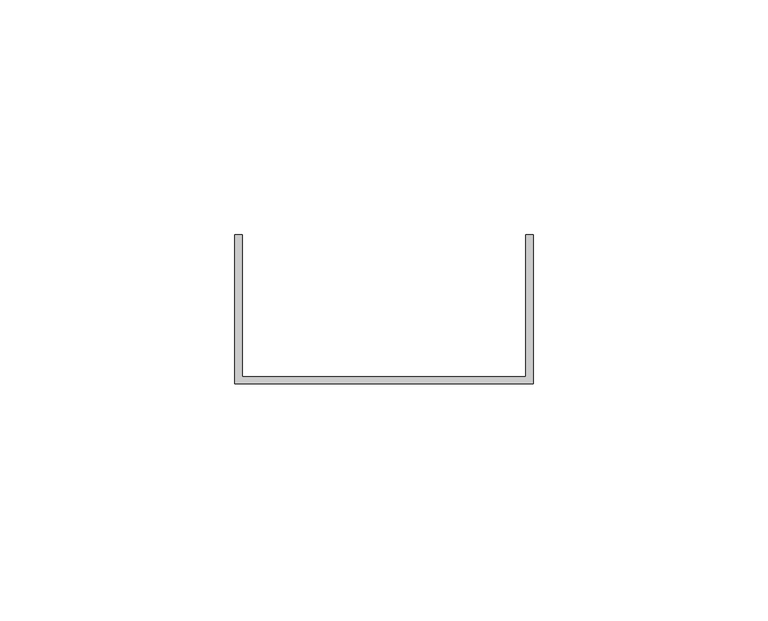
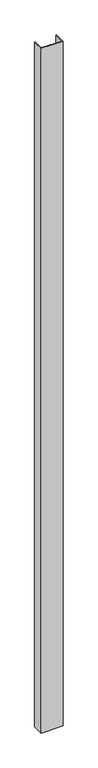
"""IFC4 building model written with IfcOpenShell, lengths in millimetres: proxy geometry, Generic Models 7:Generic Models 1:3:Generic Models 1:3 : Generic Models 7:Generic Models 1:305549:3:Generic Models 1:3:Generic Models 1:3 : Generic Models 7:Generic Models 1:305549:3 : Generic Models 7:Generic Models 1:3:Generic Models 1:3 : Generic Models 7:Generic Models 1:305549:301244:22 : Generic Models 7:Generic Models 1:3:Generic Models 1:3 : Generic Models 7:Generic Models 1:305549:3:Generic Models 1:3:Generic Models 1:3 : Generic Models 7:Generic Models 1:305549:3 : Generic Models 7:Generic Models 1:3:Generic Models 1:3 : Generic Models 7:Generic Models 1:305549:301244:308848."""

from ifc_helpers import new_model, si_unit, frame, origin, place, context, project, spatial, polyline, outline, extrude, source, transform, mapped, element, save


def generic_models_17ad937b(model_context):
    return source(origin(), model_context, "Body", "SweptSolid", [
        extrude(outline(polyline([(560352.9617239, -578753.388344), (560289.4617239, -578753.388344), (560289.4617239, -578721.638344), (560291.0492239, -578721.638344), (560291.0492239, -578751.800844), (560351.3742239, -578751.800844), (560351.3742239, -578721.638344), (560352.9617239, -578721.638344), (560352.9617239, -578753.388344)])), frame((0.0, 0.0, 4035.5735546), z_axis=(0.0, 0.0, 1.0), x_axis=(1.0, 0.0, 0.0)), (0.0, 0.0, 1.0), 2098.5264454),
    ])


if __name__ == "__main__":
    model = new_model("IFC4")
    model_context = context("Model", 3, world=origin())
    ifc_project = project(units=[si_unit("LENGTHUNIT", "METRE", prefix="MILLI")], contexts=[model_context])
    site = spatial("IfcSite", under=ifc_project)
    building = spatial("IfcBuilding", under=site)
    placement = place(None, origin())
    generic_models_shape = generic_models_17ad937b(model_context)
    element("IfcBuildingElementProxy", 1, Name="Generic Models 7:Generic Models 1:3:Generic Models 1:3 : Generic Models 7:Generic Models 1:305549:3:Generic Models 1:3:Generic Models 1:3 : Generic Models 7:Generic Models 1:305549:3 : Generic Models 7:Generic Models 1:3:Generic Models 1:3 : Generic Models 7:Generic Models 1:305549:301244:22 : Generic Models 7:Generic Models 1:3:Generic Models 1:3 : Generic Models 7:Generic Models 1:305549:3:Generic Models 1:3:Generic Models 1:3 : Generic Models 7:Generic Models 1:305549:3 : Generic Models 7:Generic Models 1:3:Generic Models 1:3 : Generic Models 7:Generic Models 1:305549:301244:308848", ObjectType="Generic Models 7:Generic Models 1:3:Generic Models 1:3 : Generic Models 7:Generic Models 1:305549:3:Generic Models 1:3:Generic Models 1:3 : Generic Models 7:Generic Models 1:305549:3 : Generic Models 7:Generic Models 1:3:Generic Models 1:3 : Generic Models 7:Generic Models 1:305549:301244:22 : Generic Models 7:Generic Models 1:3:Generic Models 1:3 : Generic Models 7:Generic Models 1:305549:3:Generic Models 1:3:Generic Models 1:3 : Generic Models 7:Generic Models 1:305549:3 : Generic Models 7:Generic Models 1:3:Generic Models 1:3 : Generic Models 7:Generic Models 1:305549:301244:308848", at=placement, inside=building, context=model_context, shape_type="MappedRepresentation", body=[
        mapped(generic_models_shape, transform((0.0, 0.0, 0.0), x_axis=(1.0, 0.0, 0.0), y_axis=(0.0, 1.0, 0.0), z_axis=(0.0, 0.0, 1.0))),
    ])
    save(model, "model.ifc")

# Revit data of these elements
# Type "Generic Models 7:Generic Models 1:3:Generic Models 1:3 : Generic Models 7:Generic Models 1:305549:3:Generic Models 1:3:Generic Models 1:3 : Generic Models 7:Generic Models 1:305549:3 : Generic Models 7:Generic Models 1:3:Generic Models 1:3 : Generic Models 7:Generic Models 1:305549:301244:22 : Generic Models 7:Generic Models 1:3:Generic Models 1:3 : Generic Models 7:Generic Models 1:305549:3:Generic Models 1:3:Generic Models 1:3 : Generic Models 7:Generic Models 1:305549:3 : Generic Models 7:Generic Models 1:3:Generic Models 1:3 : Generic Models 7:Generic Models 1:305549:301244:308848"
#   NameOverride = "Generic Models 7:Generic Models 1:3:Generic Models 1:3 : Generic Models 7:Generic Models 1:305549:3:Generic Models 1:3:Generic Models 1:3 : Generic Models 7:Generic Models 1:305549:3 : Generic Models 7:Generic Models 1:3:Generic Models 1:3 : Generic Models 7:Generic Models 1:305549:301244:308848"
#   ObjectTypeOverride = "Generic Models 1:3:Generic Models 1:3 : Generic Models 7:Generic Models 1:305549:3 : Generic Models 7:Generic Models 1:3:Generic Models 1:3 : Generic Models 7:Generic Models 1:305549:301244"
#   Reference = "Generic Models 1"
#   Tag = "308848"
# Element 1 (IfcBuildingElementProxy, "Generic Models 7:Generic Models 1:3:Generic Models 1:3 : Generic Models 7:Generic Models 1:305549:3:Generic Models 1:3:Generic Models 1:3 : Generic Models 7:Generic Models 1:305549:3 : Generic Models 7:Generic Models 1:3:Generic Models 1:3 : Generic Models 7:Generic Models 1:305549:301244:22 : Generic Models 7:Generic Models 1:3:Generic Models 1:3 : Generic Models 7:Generic Models 1:305549:3:Generic Models 1:3:Generic Models 1:3 : Generic Models 7:Generic Models 1:305549:3 : Generic Models 7:Generic Models 1:3:Generic Models 1:3 : Generic Models 7:Generic Models 1:305549:301244:308848")
#   Materials on its faces: "GALVANIZED U-CHANNEL (250T125-33)"
# Materials
#   "GALVANIZED U-CHANNEL (250T125-33)": class "Unassigned", colour RGB 202 201 200, transparency 0, Keynote = "M05451300.02", Cost = 0
